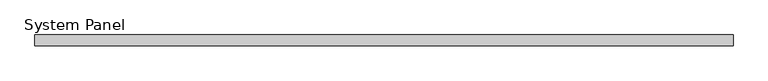
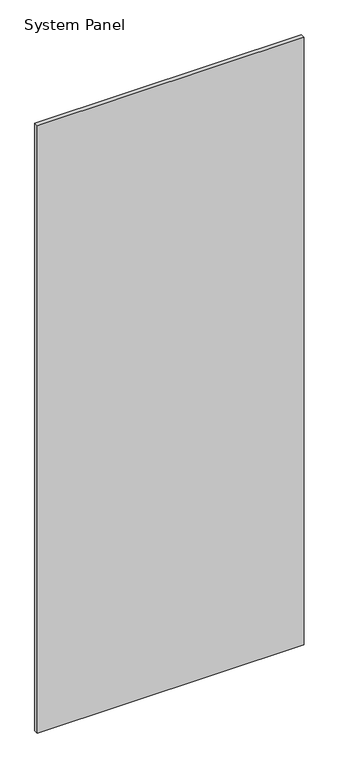
"""IFC4 building model written with IfcOpenShell, lengths in millimetres: plate geometry, System Panel : WWm-Glass-20mm-10mmOffset."""

from ifc_helpers import new_model, si_unit, origin, origin_with_axes, place, context, project, spatial, polyline, outline, extrude, source, transform, mapped, element, save


def system_panel_089d3329(model_context):
    return source(origin(), model_context, "Body", "SweptSolid", [
        extrude(outline(polyline([(655.0, 0.0), (-655.0, 0.0), (-655.0, 20.0), (655.0, 20.0), (655.0, 0.0)])), origin_with_axes(), (0.0, 0.0, 1.0), 3150.0),
    ])


if __name__ == "__main__":
    model = new_model("IFC4")
    model_context = context("Model", 3, world=origin())
    ifc_project = project(units=[si_unit("LENGTHUNIT", "METRE", prefix="MILLI")], contexts=[model_context])
    site = spatial("IfcSite", under=ifc_project)
    building = spatial("IfcBuilding", under=site)
    placement = place(None, origin())
    system_panel_shape = system_panel_089d3329(model_context)
    element("IfcPlate", 1, ObjectType="System Panel : WWm-Glass-20mm-10mmOffset", at=placement, inside=building, context=model_context, shape_type="MappedRepresentation", body=[
        mapped(system_panel_shape, transform((0.0, 0.0, 0.0), x_axis=(1.0, 0.0, 0.0), y_axis=(0.0, 1.0, 0.0), z_axis=(0.0, 0.0, 1.0))),
    ])
    save(model, "model.ifc")

# Revit data of these elements
# Type "System Panel : WWm-Glass-20mm-10mmOffset"
#   Finish = ""
# Element 1 (IfcPlate, "System Panel : WWm-Glass-20mm-10mmOffset")
#   Materials on its faces: "WW-EC-GL-Storefront"
# Materials
#   "WW-EC-GL-Storefront": class "Glass", colour RGB 236 240 239, transparency 0.85, Description = "Storefront Glass", Cost = 0
